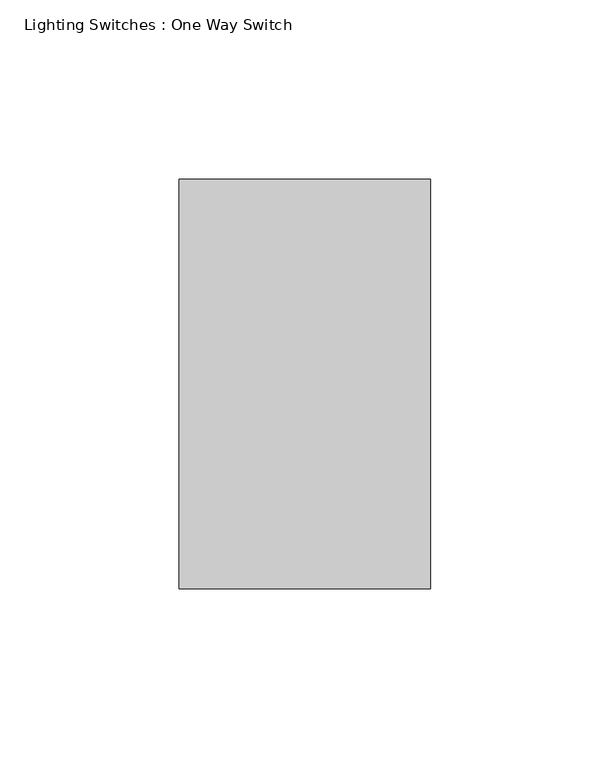
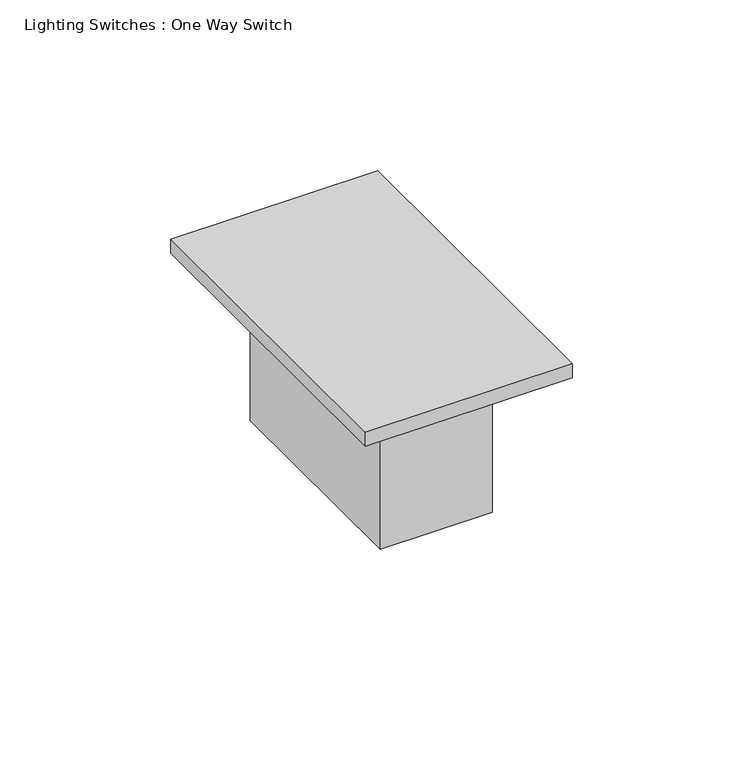
"""IFC4 building model written with IfcOpenShell, lengths in millimetres: switching device geometry, Lighting Switches : One Way Switch."""

import ifcopenshell
import ifcopenshell.guid

model = None  # the IFC model being written
_history = None  # IfcOwnerHistory: only IFC2X3 demands one
_inside = {}  # id of a spatial element -> (the spatial element, [elements in it])
_under = {}  # id of a project, library or spatial element -> (it, [spatial elements below it])
_declared = {}  # id of a project -> (the project, [libraries it declares])
_typed = {}  # id of a type object -> (the type object, [elements of that type])
_made_of = {}  # id of a material, layer set ... -> (it, [elements and type objects made of it])


def new_model(schema):
    """Start an empty IFC model of exactly this schema.

    Asked for "IFC4X3", IfcOpenShell would pick the latest addendum, in which some entities
    have other attributes; the version numbers below select the first issue.
    IFC2X3 requires an IfcOwnerHistory on every rooted entity: one is made here for all.
    """
    global model, _history
    if schema == "IFC4X3":
        model = ifcopenshell.file(schema_version=(4, 3, 0, 0))
    else:
        model = ifcopenshell.file(schema=schema)
    _inside.clear()
    _under.clear()
    _declared.clear()
    _typed.clear()
    _made_of.clear()
    _history = None
    if model.schema == "IFC2X3":
        org = make("IfcOrganization", Name="unknown")
        user = make(
            "IfcPersonAndOrganization",
            ThePerson=make("IfcPerson", FamilyName="unknown"),
            TheOrganization=org,
        )
        app = make(
            "IfcApplication",
            ApplicationDeveloper=org,
            Version="unknown",
            ApplicationFullName="unknown",
            ApplicationIdentifier="unknown",
        )
        _history = make(
            "IfcOwnerHistory",
            OwningUser=user,
            OwningApplication=app,
            ChangeAction="ADDED",
            CreationDate=0,
        )
    return model


def make(cls, **values):
    """One entity of the class cls with the attributes given. An attribute that is None is left unset."""
    return model.create_entity(
        cls, **{name: value for name, value in values.items() if value is not None}
    )


def rooted(cls, **values):
    """An entity with a GlobalId (a new one), such as an element, a storey or a relation."""
    return make(cls, GlobalId=ifcopenshell.guid.new(), OwnerHistory=_history, **values)


def si_unit(unit_type, name, prefix=None):
    """IfcSIUnit, for example si_unit("LENGTHUNIT", "METRE", prefix="MILLI")."""
    return make("IfcSIUnit", UnitType=unit_type, Prefix=prefix, Name=name)


def assignment(units):
    """IfcUnitAssignment: the units of a project."""
    return None if units is None else make("IfcUnitAssignment", Units=units)


def point(xyz):
    """IfcCartesianPoint."""
    return None if xyz is None else make("IfcCartesianPoint", Coordinates=xyz)


def direction(xyz):
    """IfcDirection."""
    return None if xyz is None else make("IfcDirection", DirectionRatios=xyz)


def frame(location, z_axis=None, x_axis=None):
    """IfcAxis2Placement3D, a coordinate frame: its origin and axes. An axis left out is left unset."""
    return make(
        "IfcAxis2Placement3D",
        Location=point(location),
        Axis=direction(z_axis),
        RefDirection=direction(x_axis),
    )


def origin():
    """The frame at (0, 0, 0) with its axes left unset."""
    return frame((0.0, 0.0, 0.0))


def origin_with_axes():
    """The frame at (0, 0, 0) with the z axis (0, 0, 1) and the x axis (1, 0, 0) written out."""
    return frame((0.0, 0.0, 0.0), z_axis=(0.0, 0.0, 1.0), x_axis=(1.0, 0.0, 0.0))


def place(relative_to, where):
    """IfcLocalPlacement: puts the frame where relative to a parent placement (None: the world)."""
    return make(
        "IfcLocalPlacement", PlacementRelTo=relative_to, RelativePlacement=where
    )


def context(
    kind, dimensions, precision=None, world=None, true_north=None, identifier=None
):
    """IfcGeometricRepresentationContext, for example the 3D "Model" context."""
    return make(
        "IfcGeometricRepresentationContext",
        ContextIdentifier=identifier,
        ContextType=kind,
        CoordinateSpaceDimension=dimensions,
        Precision=precision,
        WorldCoordinateSystem=world,
        TrueNorth=true_north,
    )


def project(units=None, contexts=None):
    """IfcProject with its units and contexts."""
    return rooted(
        "IfcProject",
        Name="project",
        RepresentationContexts=contexts,
        UnitsInContext=assignment(units),
    )


def spatial(cls, under=None, at=None, **own):
    """A site, building, storey or space (cls), placed at a placement, below another one or the project."""
    s = rooted(cls, ObjectPlacement=at, **own)
    if under is not None:
        _under.setdefault(under.id(), (under, []))[1].append(s)
    return s


def polyline(points):
    """IfcPolyline through the points."""
    return make("IfcPolyline", Points=[point(p) for p in points])


def outline(outer, holes=None, kind="AREA"):
    """IfcArbitraryClosedProfileDef: a profile drawn as a closed curve; with holes, ...WithVoids."""
    if holes is None:
        return make("IfcArbitraryClosedProfileDef", ProfileType=kind, OuterCurve=outer)
    return make(
        "IfcArbitraryProfileDefWithVoids",
        ProfileType=kind,
        OuterCurve=outer,
        InnerCurves=holes,
    )


def extrude(swept, where, along, depth):
    """IfcExtrudedAreaSolid: the profile swept, set in the frame where, extruded along a direction by depth."""
    return make(
        "IfcExtrudedAreaSolid",
        SweptArea=swept,
        Position=where,
        ExtrudedDirection=direction(along),
        Depth=depth,
    )


def shape(context_of_items, identifier, shape_type, items):
    """IfcShapeRepresentation: the items that make up one representation, for example the "Body"."""
    return make(
        "IfcShapeRepresentation",
        ContextOfItems=context_of_items,
        RepresentationIdentifier=identifier,
        RepresentationType=shape_type,
        Items=items,
    )


def source(mapping_origin, context_of_items, identifier, shape_type, items):
    """IfcRepresentationMap: a shape defined once, which mapped items show again and again."""
    return make(
        "IfcRepresentationMap",
        MappingOrigin=mapping_origin,
        MappedRepresentation=shape(context_of_items, identifier, shape_type, items),
    )


def transform(
    local_origin,
    x_axis=None,
    y_axis=None,
    z_axis=None,
    scale=None,
    scale2=None,
    scale3=None,
    uniform=True,
):
    """IfcCartesianTransformationOperator3D, or its non-uniform kind. x_axis, y_axis, z_axis: its Axis1, 2, 3."""
    if uniform:
        return make(
            "IfcCartesianTransformationOperator3D",
            Axis1=direction(x_axis),
            Axis2=direction(y_axis),
            LocalOrigin=point(local_origin),
            Scale=scale,
            Axis3=direction(z_axis),
        )
    return make(
        "IfcCartesianTransformationOperator3DnonUniform",
        Axis1=direction(x_axis),
        Axis2=direction(y_axis),
        LocalOrigin=point(local_origin),
        Scale=scale,
        Axis3=direction(z_axis),
        Scale2=scale2,
        Scale3=scale3,
    )


def mapped(mapping_source, mapping_target):
    """IfcMappedItem: shows the shape of a source again, moved by a transform."""
    return make(
        "IfcMappedItem", MappingSource=mapping_source, MappingTarget=mapping_target
    )


def made_of(thing, what):
    """Note that an element or type object is made of a material, layer set ...; save() writes the relation."""
    if what is not None:
        _made_of.setdefault(what.id(), (what, []))[1].append(thing)
    return thing


def element(
    cls,
    number,
    at=None,
    inside=None,
    cuts=None,
    type_object=None,
    material=None,
    context=None,
    identifier="Body",
    shape_type=None,
    held_by="IfcProductDefinitionShape",
    body=None,
    shapes=None,
    **own,
):
    """One element of the class cls, such as IfcWall. Its Tag is "e" and its number.

    at: its placement. inside: the storey or other place that contains it. cuts: it is an
    opening in that element (IfcRelVoidsElement). A single representation is given by context,
    identifier, shape_type and body (its items); several are given by shapes. held_by: the class
    of the entity that holds the representations. save() writes the other relations.
    """
    e = rooted(cls, Tag="e%d" % number, ObjectPlacement=at, **own)
    if body is not None:
        shapes = [shape(context, identifier, shape_type, body)]
    if shapes is not None:
        e.Representation = make(held_by, Representations=shapes)
    if inside is not None:
        _inside.setdefault(inside.id(), (inside, []))[1].append(e)
    if cuts is not None:
        rooted(
            "IfcRelVoidsElement", RelatingBuildingElement=cuts, RelatedOpeningElement=e
        )
    if type_object is not None:
        _typed.setdefault(type_object.id(), (type_object, []))[1].append(e)
    return made_of(e, material)


def aggregate(whole, parts):
    """IfcRelAggregates: a whole, such as a stair, and the parts it consists of."""
    return rooted("IfcRelAggregates", RelatingObject=whole, RelatedObjects=parts)


def save(model, path):
    """Write the relations noted so far, then the file.

    IfcRelAggregates (storeys below a building ...), IfcRelContainedInSpatialStructure (elements
    in a storey), IfcRelDefinesByType, IfcRelAssociatesMaterial and IfcRelDeclares: one each for
    every whole, place, type object, material and project.
    """
    for whole, parts in _under.values():
        aggregate(whole, parts)
    for where, things in _inside.values():
        rooted(
            "IfcRelContainedInSpatialStructure",
            RelatedElements=things,
            RelatingStructure=where,
        )
    for kind, things in _typed.values():
        rooted("IfcRelDefinesByType", RelatedObjects=things, RelatingType=kind)
    for what, things in _made_of.values():
        rooted("IfcRelAssociatesMaterial", RelatedObjects=things, RelatingMaterial=what)
    for by, libraries in _declared.values():
        rooted("IfcRelDeclares", RelatingContext=by, RelatedDefinitions=libraries)
    model.write(path)


def lighting_switches_one_way_switch_9cbd35ee(model_context):
    return source(origin(), model_context, "Body", "SweptSolid", [
        extrude(outline(polyline([(35.0, -114.0), (-35.0, -114.0), (-35.0, 0.0), (35.0, 0.0), (35.0, -114.0)])), origin_with_axes(), (0.0, 0.0, 1.0), 5.0),
        extrude(outline(polyline([(19.0, -95.0), (-19.0, -95.0), (-19.0, -19.0), (19.0, -19.0), (19.0, -95.0)])), frame((0.0, 0.0, -54.0), z_axis=(0.0, 0.0, 1.0), x_axis=(1.0, 0.0, 0.0)), (0.0, 0.0, 1.0), 54.0),
    ])


if __name__ == "__main__":
    model = new_model("IFC4")
    model_context = context("Model", 3, world=origin())
    ifc_project = project(units=[si_unit("LENGTHUNIT", "METRE", prefix="MILLI")], contexts=[model_context])
    site = spatial("IfcSite", under=ifc_project)
    building = spatial("IfcBuilding", under=site)
    placement = place(None, origin())
    lighting_switches_one_way_switch_shape = lighting_switches_one_way_switch_9cbd35ee(model_context)
    element("IfcSwitchingDevice", 1, ObjectType="Lighting Switches : One Way Switch", at=placement, inside=building, context=model_context, shape_type="MappedRepresentation", body=[
        mapped(lighting_switches_one_way_switch_shape, transform((0.0, 0.0, 0.0), x_axis=(1.0, 0.0, 0.0), y_axis=(0.0, 1.0, 0.0), z_axis=(0.0, 0.0, 1.0))),
    ])
    save(model, "model.ifc")

# Revit data of these elements
# Type "Lighting Switches : One Way Switch"
#   Label = ""
#   Width = 70 mm
#   Switch Voltage [instance default] = 230 V
#   Length = 114 mm
#   Height = 59 mm
#   Default Elevation = 1200 mm
#   Apparent Load = 0 VA
#   Visibility 7 = no
#   Visibility 6 = no
#   Visibility 5 = yes
#   Visibility 4 = no
#   Visibility 3 = no
#   Visibility 2 = no
#   Visibility 1 = no
#   Number of Poles = 1
#   Load Classification = Other
